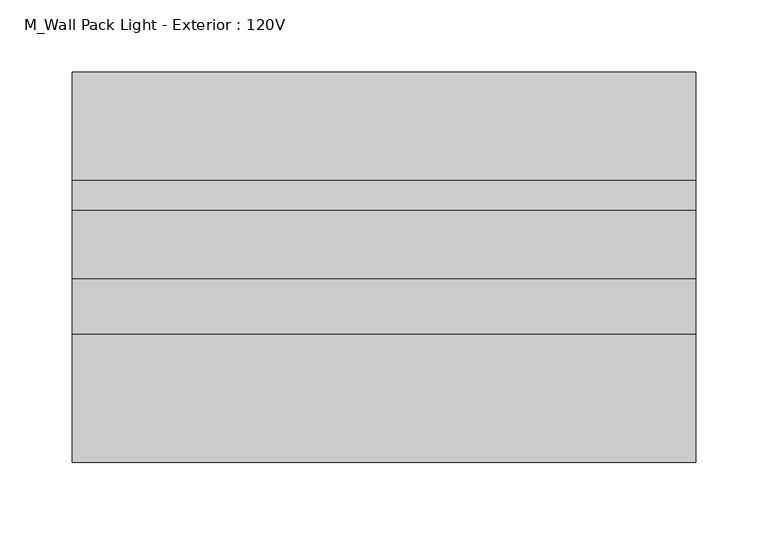
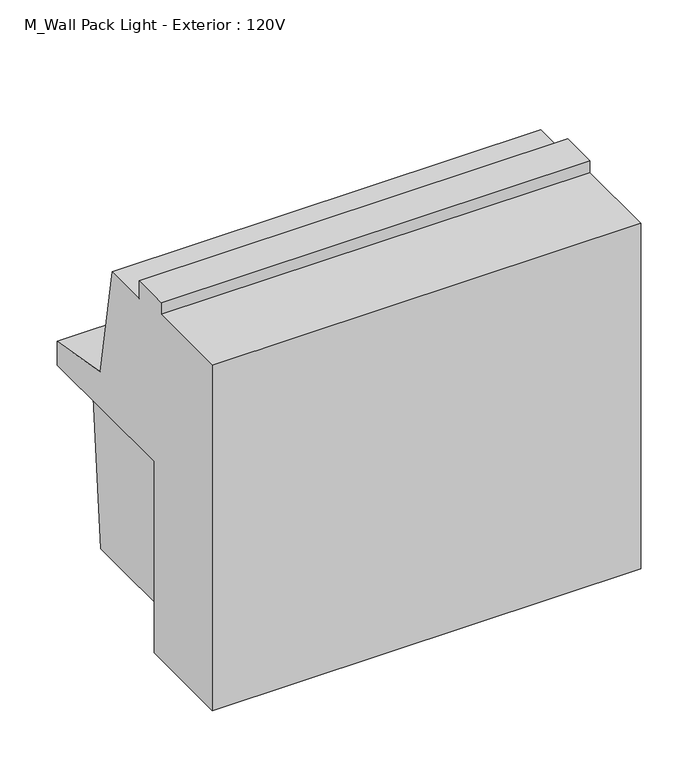
"""IFC4 building model written with IfcOpenShell, lengths in millimetres: light fixture geometry, M_Wall Pack Light - Exterior : 120V."""

from ifc_helpers import new_model, si_unit, frame, origin, place, context, project, spatial, polyline, outline, extrude, source, transform, mapped, element, save


def m_wall_pack_light_exterior_120v_7a612150(model_context):
    return source(origin(), model_context, "Body", "SweptSolid", [
        extrude(outline(polyline([(288.820745, 2350.75), (151.6, 2350.75), (151.6, 2534.9), (303.9170754, 2534.9), (288.820745, 2350.75)])), frame((-68.7349223, 0.0, 0.0), z_axis=(1.0, 0.0, 0.0), x_axis=(0.0, 1.0, 0.0)), (0.0, 0.0, 1.0), 380.9989788),
        extrude(outline(polyline([(138.9, 2712.7), (177.0, 2712.7), (177.0, 2693.65), (224.440971, 2693.65), (245.4426549, 2574.5435323), (320.4850056, 2561.3115412), (320.4850056, 2535.9115412), (151.6, 2535.9115412), (151.6, 2331.7), (50.0, 2331.7), (50.0, 2700.0), (138.9, 2700.0), (138.9, 2712.7)])), frame((-94.1359435, 0.0, 0.0), z_axis=(1.0, 0.0, 0.0), x_axis=(0.0, 1.0, 0.0)), (0.0, 0.0, 1.0), 431.8),
    ])


if __name__ == "__main__":
    model = new_model("IFC4")
    model_context = context("Model", 3, world=origin())
    ifc_project = project(units=[si_unit("LENGTHUNIT", "METRE", prefix="MILLI")], contexts=[model_context])
    site = spatial("IfcSite", under=ifc_project)
    building = spatial("IfcBuilding", under=site)
    placement = place(None, origin())
    m_wall_pack_light_exterior_120v_shape = m_wall_pack_light_exterior_120v_7a612150(model_context)
    element("IfcLightFixture", 1, ObjectType="M_Wall Pack Light - Exterior : 120V", at=placement, inside=building, context=model_context, shape_type="MappedRepresentation", body=[
        mapped(m_wall_pack_light_exterior_120v_shape, transform((0.0, 0.0, 0.0), x_axis=(1.0, 0.0, 0.0), y_axis=(0.0, 1.0, 0.0), z_axis=(0.0, 0.0, 1.0))),
    ])
    save(model, "model.ifc")

# Revit data of these elements
# Type "M_Wall Pack Light - Exterior : 120V"
#   Assembly Code = "D5020230"
#   Wattage = 70 W
#   built-in parameter 1150110 = 1 (stored number, unit not read)
#   built-in parameter 1114217 = 1 (stored number, unit not read)
#   built-in parameter 1150109 = 1 (stored number, unit not read)
#   built-in parameter 1150113 = 1 (stored number, unit not read)
#   built-in parameter 1150115 = 1 (stored number, unit not read)
#   built-in parameter 1150105 = 437.668 (stored number, unit not read)
#   Light Source Symbol Size = 609.6 mm
#   built-in parameter 1150112 = 1 (stored number, unit not read)
#   built-in parameter 1150114 = 1 (stored number, unit not read)
#   built-in parameter 1150107 = 4000 (stored number, unit not read)
#   built-in parameter 1150106 = 4.37668 (stored number, unit not read)
#   built-in parameter 1150104 = 7.29939 (stored number, unit not read)
#   Ballast Voltage = 120 V
#   built-in parameter 1114218 = 1 (stored number, unit not read)
#   built-in parameter 1150133 = 10 (stored number, unit not read)
#   Lumens = 5499.9 lm
#   Mounting Height = 2700 mm
#   Apparent Load = 70 VA
#   built-in parameter 1150134 = 12
#   built-in parameter 1150137 = 1
#   Color Filter = 16777215
#   Ballast Number of Poles = 1
#   Wall Mount Material = Metal - Paint Finish - Dark Grey, Matte
#   Shade Material = Glass
#   Load Classification = Lighting - Exterior
#   Dimming Lamp Color Temperature Shift = (empty or 0)
#   Default Elevation = 0
# Element 1 (IfcLightFixture, "M_Wall Pack Light - Exterior : 120V")
#   Materials on its faces: "Metal - Paint Finish - Dark Grey, Matte", "Glass"
# Materials
#   "Metal - Paint Finish - Dark Grey, Matte": class "Paint", colour RGB 98 98 98, transparency 0
#   "Glass": class "Glass", colour RGB 140 218 255, transparency 0.75, Description = "Soda Lime Glass", Cost = 0
